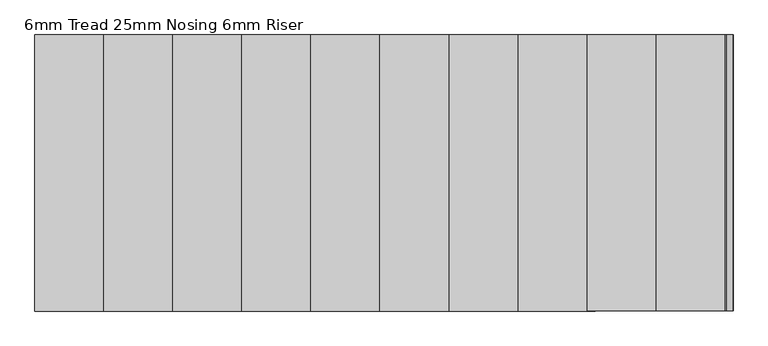
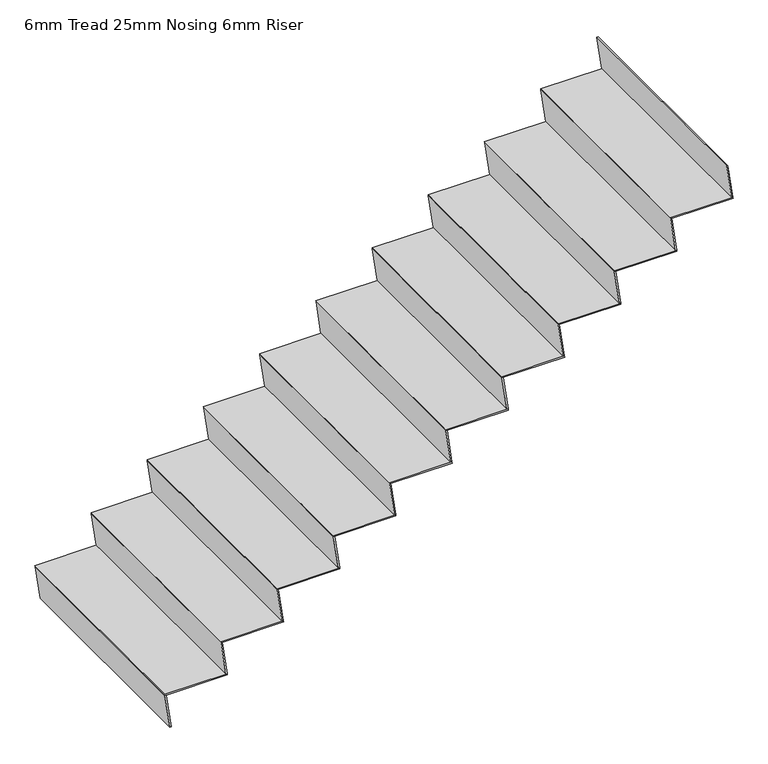
"""IFC4 building model written with IfcOpenShell, lengths in millimetres: stair flight geometry, 6mm Tread 25mm Nosing 6mm Riser."""

import ifcopenshell
import ifcopenshell.guid

model = None  # the IFC model being written
_history = None  # IfcOwnerHistory: only IFC2X3 demands one
_inside = {}  # id of a spatial element -> (the spatial element, [elements in it])
_under = {}  # id of a project, library or spatial element -> (it, [spatial elements below it])
_declared = {}  # id of a project -> (the project, [libraries it declares])
_typed = {}  # id of a type object -> (the type object, [elements of that type])
_made_of = {}  # id of a material, layer set ... -> (it, [elements and type objects made of it])


def new_model(schema):
    """Start an empty IFC model of exactly this schema.

    Asked for "IFC4X3", IfcOpenShell would pick the latest addendum, in which some entities
    have other attributes; the version numbers below select the first issue.
    IFC2X3 requires an IfcOwnerHistory on every rooted entity: one is made here for all.
    """
    global model, _history
    if schema == "IFC4X3":
        model = ifcopenshell.file(schema_version=(4, 3, 0, 0))
    else:
        model = ifcopenshell.file(schema=schema)
    _inside.clear()
    _under.clear()
    _declared.clear()
    _typed.clear()
    _made_of.clear()
    _history = None
    if model.schema == "IFC2X3":
        org = make("IfcOrganization", Name="unknown")
        user = make(
            "IfcPersonAndOrganization",
            ThePerson=make("IfcPerson", FamilyName="unknown"),
            TheOrganization=org,
        )
        app = make(
            "IfcApplication",
            ApplicationDeveloper=org,
            Version="unknown",
            ApplicationFullName="unknown",
            ApplicationIdentifier="unknown",
        )
        _history = make(
            "IfcOwnerHistory",
            OwningUser=user,
            OwningApplication=app,
            ChangeAction="ADDED",
            CreationDate=0,
        )
    return model


def make(cls, **values):
    """One entity of the class cls with the attributes given. An attribute that is None is left unset."""
    return model.create_entity(
        cls, **{name: value for name, value in values.items() if value is not None}
    )


def rooted(cls, **values):
    """An entity with a GlobalId (a new one), such as an element, a storey or a relation."""
    return make(cls, GlobalId=ifcopenshell.guid.new(), OwnerHistory=_history, **values)


def si_unit(unit_type, name, prefix=None):
    """IfcSIUnit, for example si_unit("LENGTHUNIT", "METRE", prefix="MILLI")."""
    return make("IfcSIUnit", UnitType=unit_type, Prefix=prefix, Name=name)


def assignment(units):
    """IfcUnitAssignment: the units of a project."""
    return None if units is None else make("IfcUnitAssignment", Units=units)


def point(xyz):
    """IfcCartesianPoint."""
    return None if xyz is None else make("IfcCartesianPoint", Coordinates=xyz)


def direction(xyz):
    """IfcDirection."""
    return None if xyz is None else make("IfcDirection", DirectionRatios=xyz)


def frame(location, z_axis=None, x_axis=None):
    """IfcAxis2Placement3D, a coordinate frame: its origin and axes. An axis left out is left unset."""
    return make(
        "IfcAxis2Placement3D",
        Location=point(location),
        Axis=direction(z_axis),
        RefDirection=direction(x_axis),
    )


def origin():
    """The frame at (0, 0, 0) with its axes left unset."""
    return frame((0.0, 0.0, 0.0))


def place(relative_to, where):
    """IfcLocalPlacement: puts the frame where relative to a parent placement (None: the world)."""
    return make(
        "IfcLocalPlacement", PlacementRelTo=relative_to, RelativePlacement=where
    )


def context(
    kind, dimensions, precision=None, world=None, true_north=None, identifier=None
):
    """IfcGeometricRepresentationContext, for example the 3D "Model" context."""
    return make(
        "IfcGeometricRepresentationContext",
        ContextIdentifier=identifier,
        ContextType=kind,
        CoordinateSpaceDimension=dimensions,
        Precision=precision,
        WorldCoordinateSystem=world,
        TrueNorth=true_north,
    )


def project(units=None, contexts=None):
    """IfcProject with its units and contexts."""
    return rooted(
        "IfcProject",
        Name="project",
        RepresentationContexts=contexts,
        UnitsInContext=assignment(units),
    )


def spatial(cls, under=None, at=None, **own):
    """A site, building, storey or space (cls), placed at a placement, below another one or the project."""
    s = rooted(cls, ObjectPlacement=at, **own)
    if under is not None:
        _under.setdefault(under.id(), (under, []))[1].append(s)
    return s


def polyline(points):
    """IfcPolyline through the points."""
    return make("IfcPolyline", Points=[point(p) for p in points])


def outline(outer, holes=None, kind="AREA"):
    """IfcArbitraryClosedProfileDef: a profile drawn as a closed curve; with holes, ...WithVoids."""
    if holes is None:
        return make("IfcArbitraryClosedProfileDef", ProfileType=kind, OuterCurve=outer)
    return make(
        "IfcArbitraryProfileDefWithVoids",
        ProfileType=kind,
        OuterCurve=outer,
        InnerCurves=holes,
    )


def extrude(swept, where, along, depth):
    """IfcExtrudedAreaSolid: the profile swept, set in the frame where, extruded along a direction by depth."""
    return make(
        "IfcExtrudedAreaSolid",
        SweptArea=swept,
        Position=where,
        ExtrudedDirection=direction(along),
        Depth=depth,
    )


def shape(context_of_items, identifier, shape_type, items):
    """IfcShapeRepresentation: the items that make up one representation, for example the "Body"."""
    return make(
        "IfcShapeRepresentation",
        ContextOfItems=context_of_items,
        RepresentationIdentifier=identifier,
        RepresentationType=shape_type,
        Items=items,
    )


def source(mapping_origin, context_of_items, identifier, shape_type, items):
    """IfcRepresentationMap: a shape defined once, which mapped items show again and again."""
    return make(
        "IfcRepresentationMap",
        MappingOrigin=mapping_origin,
        MappedRepresentation=shape(context_of_items, identifier, shape_type, items),
    )


def transform(
    local_origin,
    x_axis=None,
    y_axis=None,
    z_axis=None,
    scale=None,
    scale2=None,
    scale3=None,
    uniform=True,
):
    """IfcCartesianTransformationOperator3D, or its non-uniform kind. x_axis, y_axis, z_axis: its Axis1, 2, 3."""
    if uniform:
        return make(
            "IfcCartesianTransformationOperator3D",
            Axis1=direction(x_axis),
            Axis2=direction(y_axis),
            LocalOrigin=point(local_origin),
            Scale=scale,
            Axis3=direction(z_axis),
        )
    return make(
        "IfcCartesianTransformationOperator3DnonUniform",
        Axis1=direction(x_axis),
        Axis2=direction(y_axis),
        LocalOrigin=point(local_origin),
        Scale=scale,
        Axis3=direction(z_axis),
        Scale2=scale2,
        Scale3=scale3,
    )


def mapped(mapping_source, mapping_target):
    """IfcMappedItem: shows the shape of a source again, moved by a transform."""
    return make(
        "IfcMappedItem", MappingSource=mapping_source, MappingTarget=mapping_target
    )


def made_of(thing, what):
    """Note that an element or type object is made of a material, layer set ...; save() writes the relation."""
    if what is not None:
        _made_of.setdefault(what.id(), (what, []))[1].append(thing)
    return thing


def element(
    cls,
    number,
    at=None,
    inside=None,
    cuts=None,
    type_object=None,
    material=None,
    context=None,
    identifier="Body",
    shape_type=None,
    held_by="IfcProductDefinitionShape",
    body=None,
    shapes=None,
    **own,
):
    """One element of the class cls, such as IfcWall. Its Tag is "e" and its number.

    at: its placement. inside: the storey or other place that contains it. cuts: it is an
    opening in that element (IfcRelVoidsElement). A single representation is given by context,
    identifier, shape_type and body (its items); several are given by shapes. held_by: the class
    of the entity that holds the representations. save() writes the other relations.
    """
    e = rooted(cls, Tag="e%d" % number, ObjectPlacement=at, **own)
    if body is not None:
        shapes = [shape(context, identifier, shape_type, body)]
    if shapes is not None:
        e.Representation = make(held_by, Representations=shapes)
    if inside is not None:
        _inside.setdefault(inside.id(), (inside, []))[1].append(e)
    if cuts is not None:
        rooted(
            "IfcRelVoidsElement", RelatingBuildingElement=cuts, RelatedOpeningElement=e
        )
    if type_object is not None:
        _typed.setdefault(type_object.id(), (type_object, []))[1].append(e)
    return made_of(e, material)


def aggregate(whole, parts):
    """IfcRelAggregates: a whole, such as a stair, and the parts it consists of."""
    return rooted("IfcRelAggregates", RelatingObject=whole, RelatedObjects=parts)


def save(model, path):
    """Write the relations noted so far, then the file.

    IfcRelAggregates (storeys below a building ...), IfcRelContainedInSpatialStructure (elements
    in a storey), IfcRelDefinesByType, IfcRelAssociatesMaterial and IfcRelDeclares: one each for
    every whole, place, type object, material and project.
    """
    for whole, parts in _under.values():
        aggregate(whole, parts)
    for where, things in _inside.values():
        rooted(
            "IfcRelContainedInSpatialStructure",
            RelatedElements=things,
            RelatingStructure=where,
        )
    for kind, things in _typed.values():
        rooted("IfcRelDefinesByType", RelatedObjects=things, RelatingType=kind)
    for what, things in _made_of.values():
        rooted("IfcRelAssociatesMaterial", RelatedObjects=things, RelatingMaterial=what)
    for by, libraries in _declared.values():
        rooted("IfcRelDeclares", RelatingContext=by, RelatedDefinitions=libraries)
    model.write(path)


def stair_flight_6mm_tread_25mm_nosing_6mm_riser_03461877(model_context):
    return source(origin(), model_context, "Body", "SweptSolid", [
        extrude(outline(polyline([(177.7777778, 13906.0590357), (177.7777778, 13600.0), (171.7777778, 13600.84375), (171.7777778, 13906.9027857), (177.7777778, 13906.0590357)])), frame((0.0, 10370.4345331, 0.0), z_axis=(0.0, 1.0, 0.0), x_axis=(0.0, 0.0, 1.0)), (0.0, 0.0, 1.0), 1100.0),
        extrude(outline(polyline([(171.7777778, 13600.84375), (0.0, 13625.0), (0.0, 13631.0590357), (171.7777778, 13606.9027857), (171.7777778, 13600.84375)])), frame((0.0, 10370.4345331, 0.0), z_axis=(0.0, 1.0, 0.0), x_axis=(0.0, 0.0, 1.0)), (0.0, 0.0, 1.0), 1100.0),
        extrude(outline(polyline([(349.5555556, 13875.84375), (177.7777778, 13900.0), (177.7777778, 13906.0590357), (349.5555556, 13881.9027857), (349.5555556, 13875.84375)])), frame((0.0, 10370.4345331, 0.0), z_axis=(0.0, 1.0, 0.0), x_axis=(0.0, 0.0, 1.0)), (0.0, 0.0, 1.0), 1100.0),
        extrude(outline(polyline([(355.5555556, 14181.0590357), (355.5555556, 13875.0), (349.5555556, 13875.84375), (349.5555556, 14181.9027857), (355.5555556, 14181.0590357)])), frame((0.0, 10370.4345331, 0.0), z_axis=(0.0, 1.0, 0.0), x_axis=(0.0, 0.0, 1.0)), (0.0, 0.0, 1.0), 1100.0),
        extrude(outline(polyline([(527.3333333, 14150.84375), (355.5555556, 14175.0), (355.5555556, 14181.0590357), (527.3333333, 14156.9027857), (527.3333333, 14150.84375)])), frame((0.0, 10370.4345331, 0.0), z_axis=(0.0, 1.0, 0.0), x_axis=(0.0, 0.0, 1.0)), (0.0, 0.0, 1.0), 1100.0),
        extrude(outline(polyline([(533.3333333, 14456.0590357), (533.3333333, 14150.0), (527.3333333, 14150.84375), (527.3333333, 14456.9027857), (533.3333333, 14456.0590357)])), frame((0.0, 10370.4345331, 0.0), z_axis=(0.0, 1.0, 0.0), x_axis=(0.0, 0.0, 1.0)), (0.0, 0.0, 1.0), 1100.0),
        extrude(outline(polyline([(705.1111111, 14425.84375), (533.3333333, 14450.0), (533.3333333, 14456.0590357), (705.1111111, 14431.9027857), (705.1111111, 14425.84375)])), frame((0.0, 10370.4345331, 0.0), z_axis=(0.0, 1.0, 0.0), x_axis=(0.0, 0.0, 1.0)), (0.0, 0.0, 1.0), 1100.0),
        extrude(outline(polyline([(711.1111111, 14731.0590357), (711.1111111, 14425.0), (705.1111111, 14425.84375), (705.1111111, 14731.9027857), (711.1111111, 14731.0590357)])), frame((0.0, 10370.4345331, 0.0), z_axis=(0.0, 1.0, 0.0), x_axis=(0.0, 0.0, 1.0)), (0.0, 0.0, 1.0), 1100.0),
        extrude(outline(polyline([(882.8888889, 14700.84375), (711.1111111, 14725.0), (711.1111111, 14731.0590357), (882.8888889, 14706.9027857), (882.8888889, 14700.84375)])), frame((0.0, 10370.4345331, 0.0), z_axis=(0.0, 1.0, 0.0), x_axis=(0.0, 0.0, 1.0)), (0.0, 0.0, 1.0), 1100.0),
        extrude(outline(polyline([(888.8888889, 15006.0590357), (888.8888889, 14700.0), (882.8888889, 14700.84375), (882.8888889, 15006.9027857), (888.8888889, 15006.0590357)])), frame((0.0, 10370.4345331, 0.0), z_axis=(0.0, 1.0, 0.0), x_axis=(0.0, 0.0, 1.0)), (0.0, 0.0, 1.0), 1100.0),
        extrude(outline(polyline([(1060.6666667, 14975.84375), (888.8888889, 15000.0), (888.8888889, 15006.0590357), (1060.6666667, 14981.9027857), (1060.6666667, 14975.84375)])), frame((0.0, 10370.4345331, 0.0), z_axis=(0.0, 1.0, 0.0), x_axis=(0.0, 0.0, 1.0)), (0.0, 0.0, 1.0), 1100.0),
        extrude(outline(polyline([(1066.6666667, 15281.0590357), (1066.6666667, 14975.0), (1060.6666667, 14975.84375), (1060.6666667, 15281.9027857), (1066.6666667, 15281.0590357)])), frame((0.0, 10370.4345331, 0.0), z_axis=(0.0, 1.0, 0.0), x_axis=(0.0, 0.0, 1.0)), (0.0, 0.0, 1.0), 1100.0),
        extrude(outline(polyline([(1238.4444444, 15250.84375), (1066.6666667, 15275.0), (1066.6666667, 15281.0590357), (1238.4444444, 15256.9027857), (1238.4444444, 15250.84375)])), frame((0.0, 10370.4345331, 0.0), z_axis=(0.0, 1.0, 0.0), x_axis=(0.0, 0.0, 1.0)), (0.0, 0.0, 1.0), 1100.0),
        extrude(outline(polyline([(1244.4444444, 15556.0590357), (1244.4444444, 15250.0), (1238.4444444, 15250.84375), (1238.4444444, 15556.9027857), (1244.4444444, 15556.0590357)])), frame((0.0, 10370.4345331, 0.0), z_axis=(0.0, 1.0, 0.0), x_axis=(0.0, 0.0, 1.0)), (0.0, 0.0, 1.0), 1100.0),
        extrude(outline(polyline([(1416.2222222, 15525.84375), (1244.4444444, 15550.0), (1244.4444444, 15556.0590357), (1416.2222222, 15531.9027857), (1416.2222222, 15525.84375)])), frame((0.0, 10370.4345331, 0.0), z_axis=(0.0, 1.0, 0.0), x_axis=(0.0, 0.0, 1.0)), (0.0, 0.0, 1.0), 1100.0),
        extrude(outline(polyline([(1422.2222222, 15831.0590357), (1422.2222222, 15525.0), (1416.2222222, 15525.84375), (1416.2222222, 15831.9027857), (1422.2222222, 15831.0590357)])), frame((0.0, 10370.4345331, 0.0), z_axis=(0.0, 1.0, 0.0), x_axis=(0.0, 0.0, 1.0)), (0.0, 0.0, 1.0), 1100.0),
        extrude(outline(polyline([(1594.0, 15800.84375), (1422.2222222, 15825.0), (1422.2222222, 15831.0590357), (1594.0, 15806.9027857), (1594.0, 15800.84375)])), frame((0.0, 10370.4345331, 0.0), z_axis=(0.0, 1.0, 0.0), x_axis=(0.0, 0.0, 1.0)), (0.0, 0.0, 1.0), 1100.0),
        extrude(outline(polyline([(1600.0, 16106.0590357), (1600.0, 15800.0), (1594.0, 15800.84375), (1594.0, 16106.9027857), (1600.0, 16106.0590357)])), frame((0.0, 10370.4345331, 0.0), z_axis=(0.0, 1.0, 0.0), x_axis=(0.0, 0.0, 1.0)), (0.0, 0.0, 1.0), 1100.0),
        extrude(outline(polyline([(1771.7777778, 16075.84375), (1600.0, 16100.0), (1600.0, 16106.0590357), (1771.7777778, 16081.9027857), (1771.7777778, 16075.84375)])), frame((0.0, 10370.4345331, 0.0), z_axis=(0.0, 1.0, 0.0), x_axis=(0.0, 0.0, 1.0)), (0.0, 0.0, 1.0), 1100.0),
        extrude(outline(polyline([(1949.5555556, 16350.84375), (1777.7777778, 16375.0), (1777.7777778, 16381.0590357), (1949.5555556, 16356.9027857), (1949.5555556, 16350.84375)])), frame((0.0, 10370.4345331, 0.0), z_axis=(0.0, 1.0, 0.0), x_axis=(0.0, 0.0, 1.0)), (0.0, 0.0, 1.0), 1100.0),
        extrude(outline(polyline([(1777.7777778, 16381.0590357), (1777.7777778, 16075.0), (1771.7777778, 16075.84375), (1771.7777778, 16381.9027857), (1777.7777778, 16381.0590357)])), frame((0.0, 10370.4345331, 0.0), z_axis=(0.0, 1.0, 0.0), x_axis=(0.0, 0.0, 1.0)), (0.0, 0.0, 1.0), 1100.0),
    ])


if __name__ == "__main__":
    model = new_model("IFC4")
    model_context = context("Model", 3, world=origin())
    ifc_project = project(units=[si_unit("LENGTHUNIT", "METRE", prefix="MILLI")], contexts=[model_context])
    site = spatial("IfcSite", under=ifc_project)
    building = spatial("IfcBuilding", under=site)
    placement = place(None, origin())
    stair_flight_6mm_tread_25mm_nosing_6mm_riser_shape = stair_flight_6mm_tread_25mm_nosing_6mm_riser_03461877(model_context)
    element("IfcStairFlight", 1, ObjectType="6mm Tread 25mm Nosing 6mm Riser", at=placement, inside=building, context=model_context, shape_type="MappedRepresentation", body=[
        mapped(stair_flight_6mm_tread_25mm_nosing_6mm_riser_shape, transform((0.0, 0.0, 0.0), x_axis=(1.0, 0.0, 0.0), y_axis=(0.0, 1.0, 0.0), z_axis=(0.0, 0.0, 1.0))),
    ])
    save(model, "model.ifc")

# Revit data of these elements
# Element 1 (IfcStairFlight, "6mm Tread 25mm Nosing 6mm Riser")
#   Materials on its faces: "Steel, Paint Finish, Dark Gray"
# Materials
#   "Steel, Paint Finish, Dark Gray": class "Metal", colour RGB 89 89 89, transparency 0, Description = "Steel, paint finish, dark gray, glossy", Cost = 0
